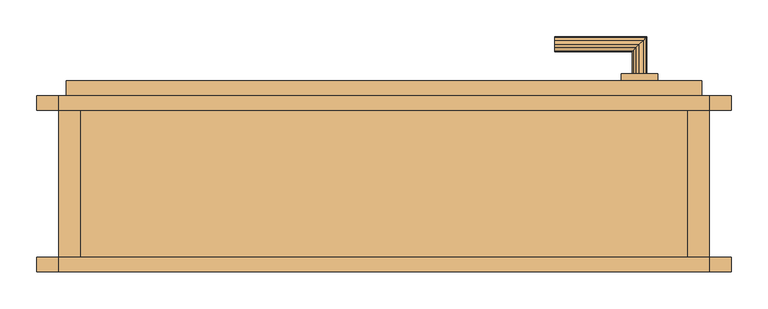
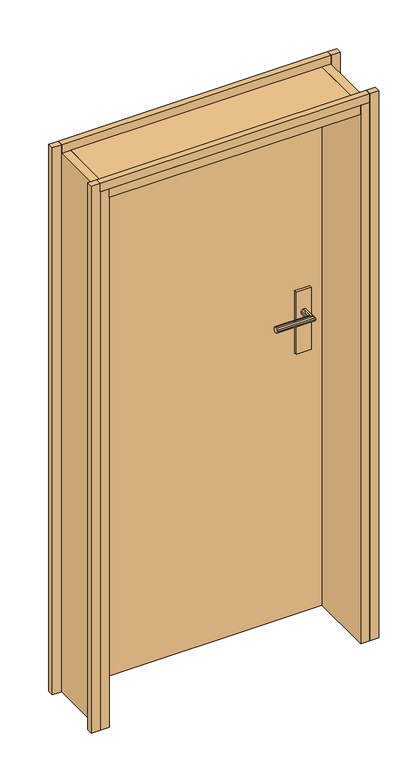
"""IFC4 building model written with IfcOpenShell, lengths in millimetres: door geometry, Tür."""

import ifcopenshell
import ifcopenshell.guid

model = None  # the IFC model being written
_history = None  # IfcOwnerHistory: only IFC2X3 demands one
_inside = {}  # id of a spatial element -> (the spatial element, [elements in it])
_under = {}  # id of a project, library or spatial element -> (it, [spatial elements below it])
_declared = {}  # id of a project -> (the project, [libraries it declares])
_typed = {}  # id of a type object -> (the type object, [elements of that type])
_made_of = {}  # id of a material, layer set ... -> (it, [elements and type objects made of it])


def new_model(schema):
    """Start an empty IFC model of exactly this schema.

    Asked for "IFC4X3", IfcOpenShell would pick the latest addendum, in which some entities
    have other attributes; the version numbers below select the first issue.
    IFC2X3 requires an IfcOwnerHistory on every rooted entity: one is made here for all.
    """
    global model, _history
    if schema == "IFC4X3":
        model = ifcopenshell.file(schema_version=(4, 3, 0, 0))
    else:
        model = ifcopenshell.file(schema=schema)
    _inside.clear()
    _under.clear()
    _declared.clear()
    _typed.clear()
    _made_of.clear()
    _history = None
    if model.schema == "IFC2X3":
        org = make("IfcOrganization", Name="unknown")
        user = make(
            "IfcPersonAndOrganization",
            ThePerson=make("IfcPerson", FamilyName="unknown"),
            TheOrganization=org,
        )
        app = make(
            "IfcApplication",
            ApplicationDeveloper=org,
            Version="unknown",
            ApplicationFullName="unknown",
            ApplicationIdentifier="unknown",
        )
        _history = make(
            "IfcOwnerHistory",
            OwningUser=user,
            OwningApplication=app,
            ChangeAction="ADDED",
            CreationDate=0,
        )
    return model


def make(cls, **values):
    """One entity of the class cls with the attributes given. An attribute that is None is left unset."""
    return model.create_entity(
        cls, **{name: value for name, value in values.items() if value is not None}
    )


def rooted(cls, **values):
    """An entity with a GlobalId (a new one), such as an element, a storey or a relation."""
    return make(cls, GlobalId=ifcopenshell.guid.new(), OwnerHistory=_history, **values)


def si_unit(unit_type, name, prefix=None):
    """IfcSIUnit, for example si_unit("LENGTHUNIT", "METRE", prefix="MILLI")."""
    return make("IfcSIUnit", UnitType=unit_type, Prefix=prefix, Name=name)


def assignment(units):
    """IfcUnitAssignment: the units of a project."""
    return None if units is None else make("IfcUnitAssignment", Units=units)


def point(xyz):
    """IfcCartesianPoint."""
    return None if xyz is None else make("IfcCartesianPoint", Coordinates=xyz)


def direction(xyz):
    """IfcDirection."""
    return None if xyz is None else make("IfcDirection", DirectionRatios=xyz)


def frame(location, z_axis=None, x_axis=None):
    """IfcAxis2Placement3D, a coordinate frame: its origin and axes. An axis left out is left unset."""
    return make(
        "IfcAxis2Placement3D",
        Location=point(location),
        Axis=direction(z_axis),
        RefDirection=direction(x_axis),
    )


def origin():
    """The frame at (0, 0, 0) with its axes left unset."""
    return frame((0.0, 0.0, 0.0))


def place(relative_to, where):
    """IfcLocalPlacement: puts the frame where relative to a parent placement (None: the world)."""
    return make(
        "IfcLocalPlacement", PlacementRelTo=relative_to, RelativePlacement=where
    )


def context(
    kind, dimensions, precision=None, world=None, true_north=None, identifier=None
):
    """IfcGeometricRepresentationContext, for example the 3D "Model" context."""
    return make(
        "IfcGeometricRepresentationContext",
        ContextIdentifier=identifier,
        ContextType=kind,
        CoordinateSpaceDimension=dimensions,
        Precision=precision,
        WorldCoordinateSystem=world,
        TrueNorth=true_north,
    )


def project(units=None, contexts=None):
    """IfcProject with its units and contexts."""
    return rooted(
        "IfcProject",
        Name="project",
        RepresentationContexts=contexts,
        UnitsInContext=assignment(units),
    )


def spatial(cls, under=None, at=None, **own):
    """A site, building, storey or space (cls), placed at a placement, below another one or the project."""
    s = rooted(cls, ObjectPlacement=at, **own)
    if under is not None:
        _under.setdefault(under.id(), (under, []))[1].append(s)
    return s


def polyline(points):
    """IfcPolyline through the points."""
    return make("IfcPolyline", Points=[point(p) for p in points])


def outline(outer, holes=None, kind="AREA"):
    """IfcArbitraryClosedProfileDef: a profile drawn as a closed curve; with holes, ...WithVoids."""
    if holes is None:
        return make("IfcArbitraryClosedProfileDef", ProfileType=kind, OuterCurve=outer)
    return make(
        "IfcArbitraryProfileDefWithVoids",
        ProfileType=kind,
        OuterCurve=outer,
        InnerCurves=holes,
    )


def extrude(swept, where, along, depth):
    """IfcExtrudedAreaSolid: the profile swept, set in the frame where, extruded along a direction by depth."""
    return make(
        "IfcExtrudedAreaSolid",
        SweptArea=swept,
        Position=where,
        ExtrudedDirection=direction(along),
        Depth=depth,
    )


def faces_of(points, faces, orient=None, outer=None):
    """IfcFace entities. A face is a list of loops; a loop is a list of indices into points, from 0.

    orient and outer hold one flag for each loop. By default every Orientation is true, the
    first loop of a face is its IfcFaceOuterBound and the others are IfcFaceBound.
    """
    made = []
    for i, loops in enumerate(faces):
        bounds = []
        for j, loop in enumerate(loops):
            is_outer = j == 0 if outer is None else outer[i][j]
            bounds.append(
                make(
                    "IfcFaceOuterBound" if is_outer else "IfcFaceBound",
                    Bound=make("IfcPolyLoop", Polygon=[points[k] for k in loop]),
                    Orientation=True if orient is None else orient[i][j],
                )
            )
        made.append(make("IfcFace", Bounds=bounds))
    return made


def faceted_brep(points, faces, orient=None, outer=None, voids=None):
    """IfcFacetedBrep: a solid bounded by flat faces; with voids (closed shells), ...WithVoids."""
    shared = [point(p) for p in points]
    hull = make("IfcClosedShell", CfsFaces=faces_of(shared, faces, orient, outer))
    if voids is None:
        return make("IfcFacetedBrep", Outer=hull)
    return make(
        "IfcFacetedBrepWithVoids",
        Outer=hull,
        Voids=[
            make(cls, CfsFaces=faces_of(shared, fs, o, b)) for cls, fs, o, b in voids
        ],
    )


def shape(context_of_items, identifier, shape_type, items):
    """IfcShapeRepresentation: the items that make up one representation, for example the "Body"."""
    return make(
        "IfcShapeRepresentation",
        ContextOfItems=context_of_items,
        RepresentationIdentifier=identifier,
        RepresentationType=shape_type,
        Items=items,
    )


def source(mapping_origin, context_of_items, identifier, shape_type, items):
    """IfcRepresentationMap: a shape defined once, which mapped items show again and again."""
    return make(
        "IfcRepresentationMap",
        MappingOrigin=mapping_origin,
        MappedRepresentation=shape(context_of_items, identifier, shape_type, items),
    )


def transform(
    local_origin,
    x_axis=None,
    y_axis=None,
    z_axis=None,
    scale=None,
    scale2=None,
    scale3=None,
    uniform=True,
):
    """IfcCartesianTransformationOperator3D, or its non-uniform kind. x_axis, y_axis, z_axis: its Axis1, 2, 3."""
    if uniform:
        return make(
            "IfcCartesianTransformationOperator3D",
            Axis1=direction(x_axis),
            Axis2=direction(y_axis),
            LocalOrigin=point(local_origin),
            Scale=scale,
            Axis3=direction(z_axis),
        )
    return make(
        "IfcCartesianTransformationOperator3DnonUniform",
        Axis1=direction(x_axis),
        Axis2=direction(y_axis),
        LocalOrigin=point(local_origin),
        Scale=scale,
        Axis3=direction(z_axis),
        Scale2=scale2,
        Scale3=scale3,
    )


def mapped(mapping_source, mapping_target):
    """IfcMappedItem: shows the shape of a source again, moved by a transform."""
    return make(
        "IfcMappedItem", MappingSource=mapping_source, MappingTarget=mapping_target
    )


def made_of(thing, what):
    """Note that an element or type object is made of a material, layer set ...; save() writes the relation."""
    if what is not None:
        _made_of.setdefault(what.id(), (what, []))[1].append(thing)
    return thing


def element(
    cls,
    number,
    at=None,
    inside=None,
    cuts=None,
    type_object=None,
    material=None,
    context=None,
    identifier="Body",
    shape_type=None,
    held_by="IfcProductDefinitionShape",
    body=None,
    shapes=None,
    **own,
):
    """One element of the class cls, such as IfcWall. Its Tag is "e" and its number.

    at: its placement. inside: the storey or other place that contains it. cuts: it is an
    opening in that element (IfcRelVoidsElement). A single representation is given by context,
    identifier, shape_type and body (its items); several are given by shapes. held_by: the class
    of the entity that holds the representations. save() writes the other relations.
    """
    e = rooted(cls, Tag="e%d" % number, ObjectPlacement=at, **own)
    if body is not None:
        shapes = [shape(context, identifier, shape_type, body)]
    if shapes is not None:
        e.Representation = make(held_by, Representations=shapes)
    if inside is not None:
        _inside.setdefault(inside.id(), (inside, []))[1].append(e)
    if cuts is not None:
        rooted(
            "IfcRelVoidsElement", RelatingBuildingElement=cuts, RelatedOpeningElement=e
        )
    if type_object is not None:
        _typed.setdefault(type_object.id(), (type_object, []))[1].append(e)
    return made_of(e, material)


def aggregate(whole, parts):
    """IfcRelAggregates: a whole, such as a stair, and the parts it consists of."""
    return rooted("IfcRelAggregates", RelatingObject=whole, RelatedObjects=parts)


def save(model, path):
    """Write the relations noted so far, then the file.

    IfcRelAggregates (storeys below a building ...), IfcRelContainedInSpatialStructure (elements
    in a storey), IfcRelDefinesByType, IfcRelAssociatesMaterial and IfcRelDeclares: one each for
    every whole, place, type object, material and project.
    """
    for whole, parts in _under.values():
        aggregate(whole, parts)
    for where, things in _inside.values():
        rooted(
            "IfcRelContainedInSpatialStructure",
            RelatedElements=things,
            RelatingStructure=where,
        )
    for kind, things in _typed.values():
        rooted("IfcRelDefinesByType", RelatedObjects=things, RelatingType=kind)
    for what, things in _made_of.values():
        rooted("IfcRelAssociatesMaterial", RelatedObjects=things, RelatingMaterial=what)
    for by, libraries in _declared.values():
        rooted("IfcRelDeclares", RelatingContext=by, RelatedDefinitions=libraries)
    model.write(path)


def door_08fc6649(model_context):
    return source(origin(), model_context, "Body", "SolidModel", [
        extrude(outline(polyline([(885.0, 0.0), (885.0, -20.0), (0.0, -20.0), (0.0, 0.0), (885.0, 0.0)])), frame((0.0, 0.0, 2010.0), z_axis=(0.0, 0.0, 1.0), x_axis=(1.0, 0.0, 0.0)), (0.0, 0.0, 1.0), 30.0),
        extrude(outline(polyline([(815.0, 250.0), (815.0, 240.0), (765.0, 240.0), (765.0, 250.0), (815.0, 250.0)])), frame((0.0, 0.0, 1050.0), z_axis=(0.0, 0.0, 1.0), x_axis=(1.0, 0.0, 0.0)), (0.0, 0.0, 1.0), 215.0),
        extrude(outline(polyline([(915.0, 0.0), (915.0, -20.0), (885.0, -20.0), (885.0, 0.0), (915.0, 0.0)])), frame((0.0, 0.0, 140.0), z_axis=(0.0, 0.0, 1.0), x_axis=(1.0, 0.0, 0.0)), (0.0, 0.0, 1.0), 1900.0),
        extrude(outline(polyline([(855.0, 220.0), (855.0, -20.0), (30.0, -20.0), (30.0, 220.0), (855.0, 220.0)])), frame((0.0, 0.0, 1980.0), z_axis=(0.0, 0.0, 1.0), x_axis=(1.0, 0.0, 0.0)), (0.0, 0.0, 1.0), 30.0),
        extrude(outline(polyline([(0.0, -20.0), (-30.0, -20.0), (-30.0, 0.0), (0.0, 0.0), (0.0, -20.0)])), frame((0.0, 0.0, 140.0), z_axis=(0.0, 0.0, 1.0), x_axis=(1.0, 0.0, 0.0)), (0.0, 0.0, 1.0), 1900.0),
        extrude(outline(polyline([(765.0, 200.0), (815.0, 200.0), (815.0, 190.0), (765.0, 190.0), (765.0, 200.0)])), frame((0.0, 0.0, 1050.0), z_axis=(0.0, 0.0, 1.0), x_axis=(1.0, 0.0, 0.0)), (0.0, 0.0, 1.0), 215.0),
        extrude(outline(polyline([(885.0, 220.0), (885.0, -20.0), (855.0, -20.0), (855.0, 220.0), (885.0, 220.0)])), frame((0.0, 0.0, 140.0), z_axis=(0.0, 0.0, 1.0), x_axis=(1.0, 0.0, 0.0)), (0.0, 0.0, 1.0), 1870.0),
        faceted_brep([(795.0, 250.0, 1198.660254), (790.0, 250.0, 1200.0), (785.0, 250.0, 1198.660254), (781.339746, 250.0, 1195.0), (780.0, 250.0, 1190.0), (781.339746, 250.0, 1185.0), (785.0, 250.0, 1181.339746), (790.0, 250.0, 1180.0), (795.0, 250.0, 1181.339746), (798.660254, 250.0, 1185.0), (800.0, 250.0, 1190.0), (798.660254, 250.0, 1195.0), (790.0, 290.0, 1200.0), (795.0, 295.0, 1198.660254), (798.660254, 298.660254, 1195.0), (800.0, 300.0, 1190.0), (798.660254, 298.660254, 1185.0), (795.0, 295.0, 1181.339746), (790.0, 290.0, 1180.0), (785.0, 285.0, 1181.339746), (781.339746, 281.339746, 1185.0), (780.0, 280.0, 1190.0), (781.339746, 281.339746, 1195.0), (785.0, 285.0, 1198.660254), (675.0, 285.0, 1198.660254), (675.0, 290.0, 1200.0), (675.0, 295.0, 1198.660254), (675.0, 298.660254, 1195.0), (675.0, 300.0, 1190.0), (675.0, 298.660254, 1185.0), (675.0, 295.0, 1181.339746), (675.0, 290.0, 1180.0), (675.0, 285.0, 1181.339746), (675.0, 281.339746, 1185.0), (675.0, 280.0, 1190.0), (675.0, 281.339746, 1195.0)], [[[0, 1, 2, 3, 4, 5, 6, 7, 8, 9, 10, 11]], [[12, 1, 0, 13]], [[13, 0, 11, 14]], [[14, 11, 10, 15]], [[15, 10, 9, 16]], [[16, 9, 8, 17]], [[17, 8, 7, 18]], [[18, 7, 6, 19]], [[19, 6, 5, 20]], [[20, 5, 4, 21]], [[21, 4, 3, 22]], [[22, 3, 2, 23]], [[23, 2, 1, 12]], [[24, 25, 26, 27, 28, 29, 30, 31, 32, 33, 34, 35]], [[25, 12, 13, 26]], [[26, 13, 14, 27]], [[27, 14, 15, 28]], [[28, 15, 16, 29]], [[29, 16, 17, 30]], [[30, 17, 18, 31]], [[31, 18, 19, 32]], [[32, 19, 20, 33]], [[33, 20, 21, 34]], [[34, 21, 22, 35]], [[35, 22, 23, 24]], [[24, 23, 12, 25]]]),
        extrude(outline(polyline([(885.0, 220.0), (885.0, 200.0), (0.0, 200.0), (0.0, 220.0), (885.0, 220.0)])), frame((0.0, 0.0, 2010.0), z_axis=(0.0, 0.0, 1.0), x_axis=(1.0, 0.0, 0.0)), (0.0, 0.0, 1.0), 30.0),
        extrude(outline(polyline([(875.0, 240.0), (875.0, 200.0), (10.0, 200.0), (10.0, 240.0), (875.0, 240.0)])), frame((0.0, 0.0, 140.0), z_axis=(0.0, 0.0, 1.0), x_axis=(1.0, 0.0, 0.0)), (0.0, 0.0, 1.0), 1860.0),
        extrude(outline(polyline([(0.0, 200.0), (-30.0, 200.0), (-30.0, 220.0), (0.0, 220.0), (0.0, 200.0)])), frame((0.0, 0.0, 140.0), z_axis=(0.0, 0.0, 1.0), x_axis=(1.0, 0.0, 0.0)), (0.0, 0.0, 1.0), 1900.0),
        faceted_brep([(785.0, 190.0, 1198.660254), (790.0, 190.0, 1200.0), (795.0, 190.0, 1198.660254), (798.660254, 190.0, 1195.0), (800.0, 190.0, 1190.0), (798.660254, 190.0, 1185.0), (795.0, 190.0, 1181.339746), (790.0, 190.0, 1180.0), (785.0, 190.0, 1181.339746), (781.339746, 190.0, 1185.0), (780.0, 190.0, 1190.0), (781.339746, 190.0, 1195.0), (790.0, 150.0, 1200.0), (795.0, 145.0, 1198.660254), (798.660254, 141.339746, 1195.0), (800.0, 140.0, 1190.0), (798.660254, 141.339746, 1185.0), (795.0, 145.0, 1181.339746), (790.0, 150.0, 1180.0), (785.0, 155.0, 1181.339746), (781.339746, 158.660254, 1185.0), (780.0, 160.0, 1190.0), (781.339746, 158.660254, 1195.0), (785.0, 155.0, 1198.660254), (675.0, 145.0, 1198.660254), (675.0, 150.0, 1200.0), (675.0, 155.0, 1198.660254), (675.0, 158.660254, 1195.0), (675.0, 160.0, 1190.0), (675.0, 158.660254, 1185.0), (675.0, 155.0, 1181.339746), (675.0, 150.0, 1180.0), (675.0, 145.0, 1181.339746), (675.0, 141.339746, 1185.0), (675.0, 140.0, 1190.0), (675.0, 141.339746, 1195.0)], [[[0, 1, 2, 3, 4, 5, 6, 7, 8, 9, 10, 11]], [[2, 1, 12, 13]], [[3, 2, 13, 14]], [[4, 3, 14, 15]], [[5, 4, 15, 16]], [[6, 5, 16, 17]], [[7, 6, 17, 18]], [[8, 7, 18, 19]], [[9, 8, 19, 20]], [[10, 9, 20, 21]], [[11, 10, 21, 22]], [[0, 11, 22, 23]], [[1, 0, 23, 12]], [[24, 25, 26, 27, 28, 29, 30, 31, 32, 33, 34, 35]], [[13, 12, 25, 24]], [[14, 13, 24, 35]], [[15, 14, 35, 34]], [[16, 15, 34, 33]], [[17, 16, 33, 32]], [[18, 17, 32, 31]], [[19, 18, 31, 30]], [[20, 19, 30, 29]], [[21, 20, 29, 28]], [[22, 21, 28, 27]], [[23, 22, 27, 26]], [[12, 23, 26, 25]]]),
        extrude(outline(polyline([(915.0, 220.0), (915.0, 200.0), (885.0, 200.0), (885.0, 220.0), (915.0, 220.0)])), frame((0.0, 0.0, 140.0), z_axis=(0.0, 0.0, 1.0), x_axis=(1.0, 0.0, 0.0)), (0.0, 0.0, 1.0), 1900.0),
        extrude(outline(polyline([(30.0, 220.0), (30.0, -20.0), (0.0, -20.0), (0.0, 220.0), (30.0, 220.0)])), frame((0.0, 0.0, 140.0), z_axis=(0.0, 0.0, 1.0), x_axis=(1.0, 0.0, 0.0)), (0.0, 0.0, 1.0), 1870.0),
    ])


if __name__ == "__main__":
    model = new_model("IFC4")
    model_context = context("Model", 3, world=origin())
    ifc_project = project(units=[si_unit("LENGTHUNIT", "METRE", prefix="MILLI")], contexts=[model_context])
    site = spatial("IfcSite", under=ifc_project)
    building = spatial("IfcBuilding", under=site)
    placement = place(None, origin())
    door_shape = door_08fc6649(model_context)
    element("IfcDoor", 1, ObjectType="Tür", at=placement, inside=building, context=model_context, shape_type="MappedRepresentation", body=[
        mapped(door_shape, transform((0.0, 0.0, 0.0), x_axis=(1.0, 0.0, 0.0), y_axis=(0.0, 1.0, 0.0), z_axis=(0.0, 0.0, 1.0))),
    ])
    save(model, "model.ifc")

# Revit data of these elements
# Type "Tür"
#   Type Mark = "41"
# Element 1 (IfcDoor, "Tür")
#   Materials on its faces: "tuer_beschlag", "tuer_holzzarge"
# Materials
#   "tuer_beschlag": class "Unassigned", colour RGB 128 128 128, transparency 0
#   "tuer_holzzarge": class "Unassigned", colour RGB 255 255 255, transparency 0
